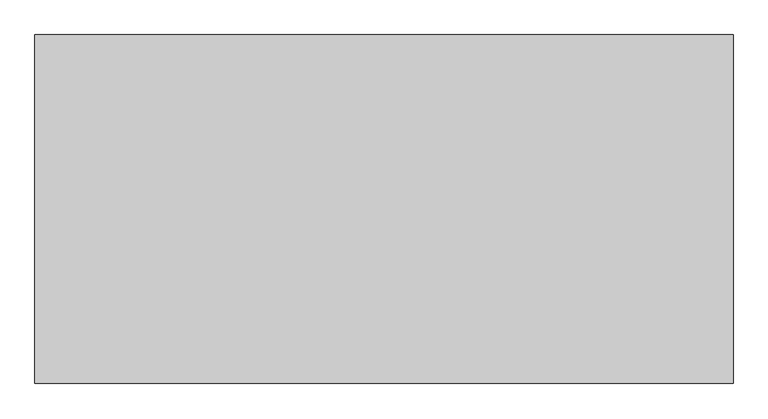
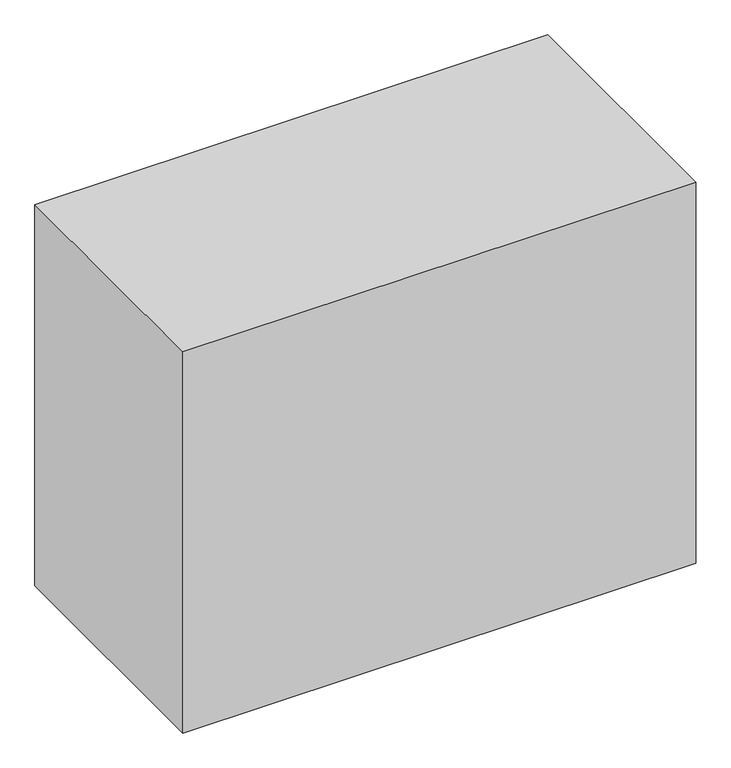
"""IFC4 building model written with IfcOpenShell, lengths in millimetres: proxy geometry, Space Planning Box_hec : Space Planning Box_hec."""

import ifcopenshell
import ifcopenshell.guid

model = None  # the IFC model being written
_history = None  # IfcOwnerHistory: only IFC2X3 demands one
_inside = {}  # id of a spatial element -> (the spatial element, [elements in it])
_under = {}  # id of a project, library or spatial element -> (it, [spatial elements below it])
_declared = {}  # id of a project -> (the project, [libraries it declares])
_typed = {}  # id of a type object -> (the type object, [elements of that type])
_made_of = {}  # id of a material, layer set ... -> (it, [elements and type objects made of it])


def new_model(schema):
    """Start an empty IFC model of exactly this schema.

    Asked for "IFC4X3", IfcOpenShell would pick the latest addendum, in which some entities
    have other attributes; the version numbers below select the first issue.
    IFC2X3 requires an IfcOwnerHistory on every rooted entity: one is made here for all.
    """
    global model, _history
    if schema == "IFC4X3":
        model = ifcopenshell.file(schema_version=(4, 3, 0, 0))
    else:
        model = ifcopenshell.file(schema=schema)
    _inside.clear()
    _under.clear()
    _declared.clear()
    _typed.clear()
    _made_of.clear()
    _history = None
    if model.schema == "IFC2X3":
        org = make("IfcOrganization", Name="unknown")
        user = make(
            "IfcPersonAndOrganization",
            ThePerson=make("IfcPerson", FamilyName="unknown"),
            TheOrganization=org,
        )
        app = make(
            "IfcApplication",
            ApplicationDeveloper=org,
            Version="unknown",
            ApplicationFullName="unknown",
            ApplicationIdentifier="unknown",
        )
        _history = make(
            "IfcOwnerHistory",
            OwningUser=user,
            OwningApplication=app,
            ChangeAction="ADDED",
            CreationDate=0,
        )
    return model


def make(cls, **values):
    """One entity of the class cls with the attributes given. An attribute that is None is left unset."""
    return model.create_entity(
        cls, **{name: value for name, value in values.items() if value is not None}
    )


def rooted(cls, **values):
    """An entity with a GlobalId (a new one), such as an element, a storey or a relation."""
    return make(cls, GlobalId=ifcopenshell.guid.new(), OwnerHistory=_history, **values)


def si_unit(unit_type, name, prefix=None):
    """IfcSIUnit, for example si_unit("LENGTHUNIT", "METRE", prefix="MILLI")."""
    return make("IfcSIUnit", UnitType=unit_type, Prefix=prefix, Name=name)


def assignment(units):
    """IfcUnitAssignment: the units of a project."""
    return None if units is None else make("IfcUnitAssignment", Units=units)


def point(xyz):
    """IfcCartesianPoint."""
    return None if xyz is None else make("IfcCartesianPoint", Coordinates=xyz)


def direction(xyz):
    """IfcDirection."""
    return None if xyz is None else make("IfcDirection", DirectionRatios=xyz)


def frame(location, z_axis=None, x_axis=None):
    """IfcAxis2Placement3D, a coordinate frame: its origin and axes. An axis left out is left unset."""
    return make(
        "IfcAxis2Placement3D",
        Location=point(location),
        Axis=direction(z_axis),
        RefDirection=direction(x_axis),
    )


def origin():
    """The frame at (0, 0, 0) with its axes left unset."""
    return frame((0.0, 0.0, 0.0))


def origin_with_axes():
    """The frame at (0, 0, 0) with the z axis (0, 0, 1) and the x axis (1, 0, 0) written out."""
    return frame((0.0, 0.0, 0.0), z_axis=(0.0, 0.0, 1.0), x_axis=(1.0, 0.0, 0.0))


def place(relative_to, where):
    """IfcLocalPlacement: puts the frame where relative to a parent placement (None: the world)."""
    return make(
        "IfcLocalPlacement", PlacementRelTo=relative_to, RelativePlacement=where
    )


def context(
    kind, dimensions, precision=None, world=None, true_north=None, identifier=None
):
    """IfcGeometricRepresentationContext, for example the 3D "Model" context."""
    return make(
        "IfcGeometricRepresentationContext",
        ContextIdentifier=identifier,
        ContextType=kind,
        CoordinateSpaceDimension=dimensions,
        Precision=precision,
        WorldCoordinateSystem=world,
        TrueNorth=true_north,
    )


def project(units=None, contexts=None):
    """IfcProject with its units and contexts."""
    return rooted(
        "IfcProject",
        Name="project",
        RepresentationContexts=contexts,
        UnitsInContext=assignment(units),
    )


def spatial(cls, under=None, at=None, **own):
    """A site, building, storey or space (cls), placed at a placement, below another one or the project."""
    s = rooted(cls, ObjectPlacement=at, **own)
    if under is not None:
        _under.setdefault(under.id(), (under, []))[1].append(s)
    return s


def polyline(points):
    """IfcPolyline through the points."""
    return make("IfcPolyline", Points=[point(p) for p in points])


def outline(outer, holes=None, kind="AREA"):
    """IfcArbitraryClosedProfileDef: a profile drawn as a closed curve; with holes, ...WithVoids."""
    if holes is None:
        return make("IfcArbitraryClosedProfileDef", ProfileType=kind, OuterCurve=outer)
    return make(
        "IfcArbitraryProfileDefWithVoids",
        ProfileType=kind,
        OuterCurve=outer,
        InnerCurves=holes,
    )


def extrude(swept, where, along, depth):
    """IfcExtrudedAreaSolid: the profile swept, set in the frame where, extruded along a direction by depth."""
    return make(
        "IfcExtrudedAreaSolid",
        SweptArea=swept,
        Position=where,
        ExtrudedDirection=direction(along),
        Depth=depth,
    )


def shape(context_of_items, identifier, shape_type, items):
    """IfcShapeRepresentation: the items that make up one representation, for example the "Body"."""
    return make(
        "IfcShapeRepresentation",
        ContextOfItems=context_of_items,
        RepresentationIdentifier=identifier,
        RepresentationType=shape_type,
        Items=items,
    )


def source(mapping_origin, context_of_items, identifier, shape_type, items):
    """IfcRepresentationMap: a shape defined once, which mapped items show again and again."""
    return make(
        "IfcRepresentationMap",
        MappingOrigin=mapping_origin,
        MappedRepresentation=shape(context_of_items, identifier, shape_type, items),
    )


def transform(
    local_origin,
    x_axis=None,
    y_axis=None,
    z_axis=None,
    scale=None,
    scale2=None,
    scale3=None,
    uniform=True,
):
    """IfcCartesianTransformationOperator3D, or its non-uniform kind. x_axis, y_axis, z_axis: its Axis1, 2, 3."""
    if uniform:
        return make(
            "IfcCartesianTransformationOperator3D",
            Axis1=direction(x_axis),
            Axis2=direction(y_axis),
            LocalOrigin=point(local_origin),
            Scale=scale,
            Axis3=direction(z_axis),
        )
    return make(
        "IfcCartesianTransformationOperator3DnonUniform",
        Axis1=direction(x_axis),
        Axis2=direction(y_axis),
        LocalOrigin=point(local_origin),
        Scale=scale,
        Axis3=direction(z_axis),
        Scale2=scale2,
        Scale3=scale3,
    )


def mapped(mapping_source, mapping_target):
    """IfcMappedItem: shows the shape of a source again, moved by a transform."""
    return make(
        "IfcMappedItem", MappingSource=mapping_source, MappingTarget=mapping_target
    )


def made_of(thing, what):
    """Note that an element or type object is made of a material, layer set ...; save() writes the relation."""
    if what is not None:
        _made_of.setdefault(what.id(), (what, []))[1].append(thing)
    return thing


def element(
    cls,
    number,
    at=None,
    inside=None,
    cuts=None,
    type_object=None,
    material=None,
    context=None,
    identifier="Body",
    shape_type=None,
    held_by="IfcProductDefinitionShape",
    body=None,
    shapes=None,
    **own,
):
    """One element of the class cls, such as IfcWall. Its Tag is "e" and its number.

    at: its placement. inside: the storey or other place that contains it. cuts: it is an
    opening in that element (IfcRelVoidsElement). A single representation is given by context,
    identifier, shape_type and body (its items); several are given by shapes. held_by: the class
    of the entity that holds the representations. save() writes the other relations.
    """
    e = rooted(cls, Tag="e%d" % number, ObjectPlacement=at, **own)
    if body is not None:
        shapes = [shape(context, identifier, shape_type, body)]
    if shapes is not None:
        e.Representation = make(held_by, Representations=shapes)
    if inside is not None:
        _inside.setdefault(inside.id(), (inside, []))[1].append(e)
    if cuts is not None:
        rooted(
            "IfcRelVoidsElement", RelatingBuildingElement=cuts, RelatedOpeningElement=e
        )
    if type_object is not None:
        _typed.setdefault(type_object.id(), (type_object, []))[1].append(e)
    return made_of(e, material)


def aggregate(whole, parts):
    """IfcRelAggregates: a whole, such as a stair, and the parts it consists of."""
    return rooted("IfcRelAggregates", RelatingObject=whole, RelatedObjects=parts)


def save(model, path):
    """Write the relations noted so far, then the file.

    IfcRelAggregates (storeys below a building ...), IfcRelContainedInSpatialStructure (elements
    in a storey), IfcRelDefinesByType, IfcRelAssociatesMaterial and IfcRelDeclares: one each for
    every whole, place, type object, material and project.
    """
    for whole, parts in _under.values():
        aggregate(whole, parts)
    for where, things in _inside.values():
        rooted(
            "IfcRelContainedInSpatialStructure",
            RelatedElements=things,
            RelatingStructure=where,
        )
    for kind, things in _typed.values():
        rooted("IfcRelDefinesByType", RelatedObjects=things, RelatingType=kind)
    for what, things in _made_of.values():
        rooted("IfcRelAssociatesMaterial", RelatedObjects=things, RelatingMaterial=what)
    for by, libraries in _declared.values():
        rooted("IfcRelDeclares", RelatingContext=by, RelatedDefinitions=libraries)
    model.write(path)


def generic_models_85ff21bb(model_context):
    return source(origin(), model_context, "Body", "SweptSolid", [
        extrude(outline(polyline([(3500.0, 1750.0), (3500.0, -1750.0), (-3500.0, -1750.0), (-3500.0, 1750.0), (3500.0, 1750.0)])), origin_with_axes(), (0.0, 0.0, 1.0), 5500.0),
    ])


if __name__ == "__main__":
    model = new_model("IFC4")
    model_context = context("Model", 3, world=origin())
    ifc_project = project(units=[si_unit("LENGTHUNIT", "METRE", prefix="MILLI")], contexts=[model_context])
    site = spatial("IfcSite", under=ifc_project)
    building = spatial("IfcBuilding", under=site)
    placement = place(None, origin())
    generic_models_shape = generic_models_85ff21bb(model_context)
    element("IfcBuildingElementProxy", 1, Name="Space Planning Box_hec : Space Planning Box_hec", ObjectType="Space Planning Box_hec : Space Planning Box_hec", at=placement, inside=building, context=model_context, shape_type="MappedRepresentation", body=[
        mapped(generic_models_shape, transform((0.0, 0.0, 0.0), x_axis=(1.0, 0.0, 0.0), y_axis=(0.0, 1.0, 0.0), z_axis=(0.0, 0.0, 1.0))),
    ])
    save(model, "model.ifc")

# Revit data of these elements
# Type "Space Planning Box_hec : Space Planning Box_hec"
#   Type Comments = "..."
#   Room Name [instance default] = "?"
#   Interior Finish [instance default] = ""
#   Exterior Finish [instance default] = ""
#   Department [instance default] = ""
#   Assembly Code = "..."
#   ceiling height [instance default] = 0
#   Width [instance default] = 1524 mm
#   Program Area [instance default] = 0.00 m²
#   Length [instance default] = 1524 mm
#   Height [instance default] = 1524 mm
#   Area [instance default] = 2.32258 m²
#   Fill Color [instance default] = Cyan
#   Default Elevation = 0
# Element 1 (IfcBuildingElementProxy, "Space Planning Box_hec : Space Planning Box_hec")
#   Room Name = "Computer Room"
#   Exterior Finish = "N/A..N/A,,EW2..N/A..N/A"
#   Department = "AR"
#   Width = 7000 mm
#   Program Area = 24.50 m²
#   Length = 3500 mm
#   Height = 5500 mm
#   Area = 24.50 m²
#   Materials on its faces: "Cyan"
# Materials
#   "Cyan": class "Generic", colour RGB 0 255 255, transparency 0.2, Cost = 0
